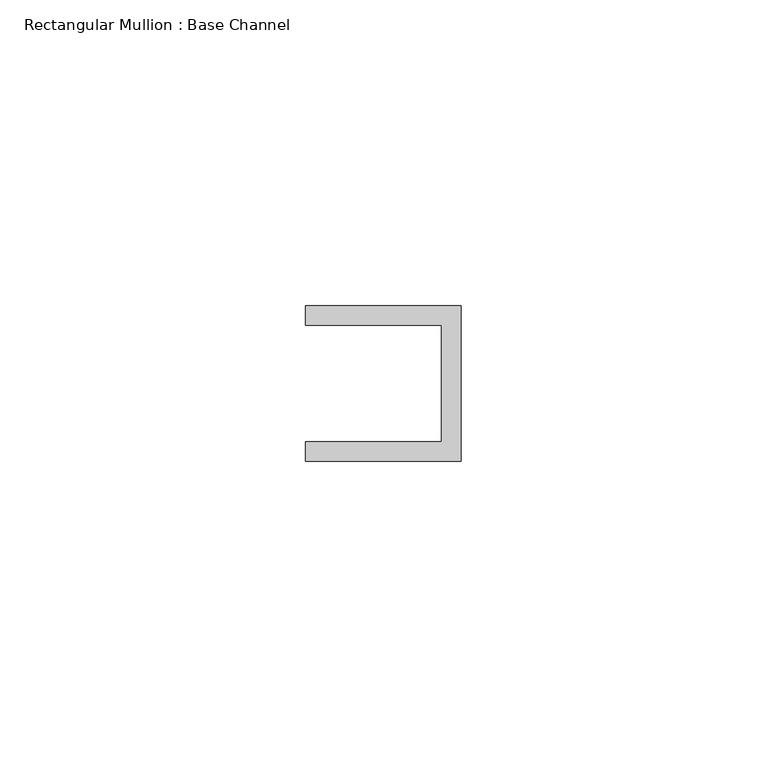
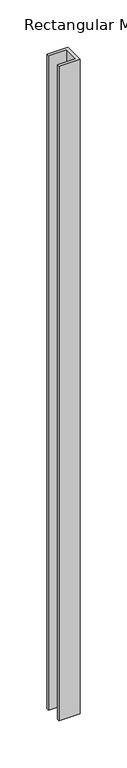
"""IFC4 building model written with IfcOpenShell, lengths in millimetres: member geometry, Rectangular Mullion : Base Channel."""

from ifc_helpers import new_model, si_unit, frame, origin, place, context, project, spatial, polyline, outline, extrude, source, transform, mapped, element, save


def rectangular_mullion_base_channel_0eca6ec0(model_context):
    return source(origin(), model_context, "Body", "SweptSolid", [
        extrude(outline(polyline([(0.0, -12.7), (-25.4, -12.7), (-25.4, -9.525), (-3.175, -9.525), (-3.175, 9.525), (-25.4, 9.525), (-25.4, 12.7), (0.0, 12.7), (0.0, -12.7)])), frame((0.0, 0.0, -845.4185495), z_axis=(0.0, 0.0, 1.0), x_axis=(1.0, 0.0, 0.0)), (0.0, 0.0, 1.0), 845.4185495),
    ])


if __name__ == "__main__":
    model = new_model("IFC4")
    model_context = context("Model", 3, world=origin())
    ifc_project = project(units=[si_unit("LENGTHUNIT", "METRE", prefix="MILLI")], contexts=[model_context])
    site = spatial("IfcSite", under=ifc_project)
    building = spatial("IfcBuilding", under=site)
    placement = place(None, origin())
    rectangular_mullion_base_channel_shape = rectangular_mullion_base_channel_0eca6ec0(model_context)
    element("IfcMember", 1, ObjectType="Rectangular Mullion : Base Channel", at=placement, inside=building, context=model_context, shape_type="MappedRepresentation", body=[
        mapped(rectangular_mullion_base_channel_shape, transform((0.0, 0.0, 0.0), x_axis=(1.0, 0.0, 0.0), y_axis=(0.0, 1.0, 0.0), z_axis=(0.0, 0.0, 1.0))),
    ])
    save(model, "model.ifc")

# Revit data of these elements
# Type "Rectangular Mullion : Base Channel"
#   built-in parameter 1007322 = 0.0833333 (stored number, unit not read)
#   built-in parameter 1007321 = 0.0416667 (stored number, unit not read)
#   built-in parameter 1007320 = -0.03125 (stored number, unit not read)
# Element 1 (IfcMember, "Rectangular Mullion : Base Channel")
#   Materials on its faces: "ALUM"
# Materials
#   "ALUM": class "Generic", colour RGB 157 157 157, transparency 0, Cost = 0
